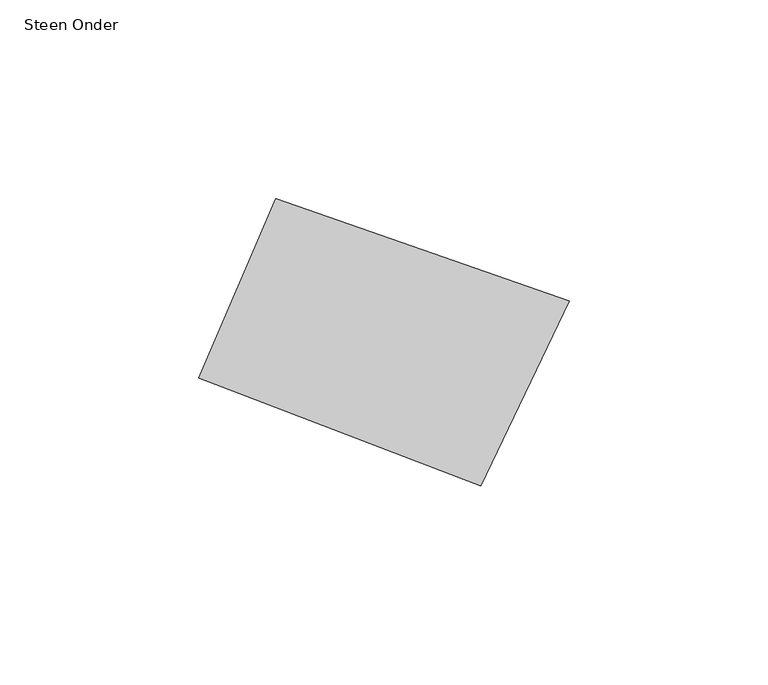
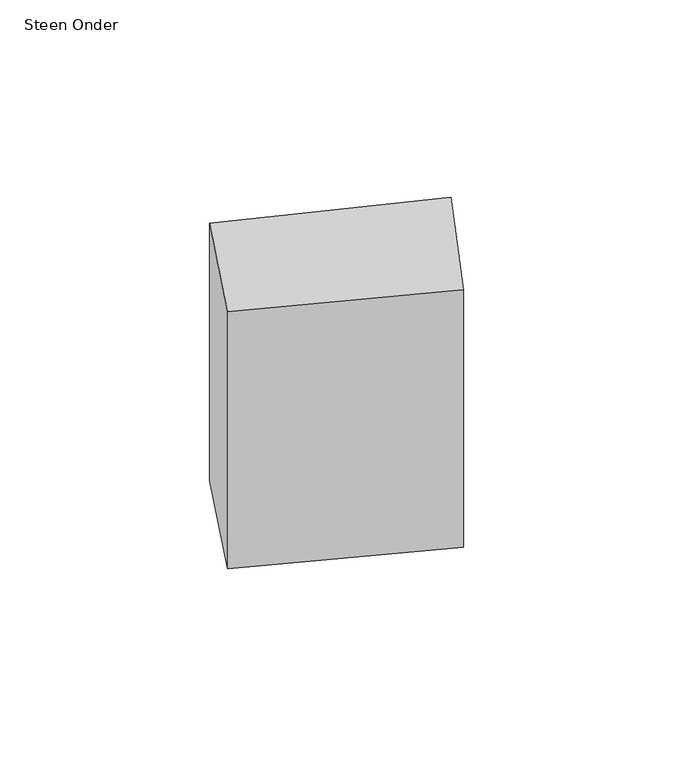
"""IFC4 building model written with IfcOpenShell, lengths in millimetres: proxy geometry, 00_GMA_steen_versie_4 : Steen Onder."""

from ifc_helpers import new_model, si_unit, frame, origin, place, context, project, spatial, polyline, outline, extrude, source, transform, mapped, element, save


def steen_onder_1c1f4d6d(model_context):
    return source(origin(), model_context, "Body", "SweptSolid", [
        extrude(outline(polyline([(138.2153403, 51.911045), (115.9401022, 5.2313815), (44.8164561, 32.4357612), (64.2804449, 77.7242813), (138.2153403, 51.911045)])), frame((0.0, 0.0, -100.0), z_axis=(0.0, 0.0, 1.0), x_axis=(1.0, 0.0, 0.0)), (0.0, 0.0, 1.0), 100.0),
    ])


if __name__ == "__main__":
    model = new_model("IFC4")
    model_context = context("Model", 3, world=origin())
    ifc_project = project(units=[si_unit("LENGTHUNIT", "METRE", prefix="MILLI")], contexts=[model_context])
    site = spatial("IfcSite", under=ifc_project)
    building = spatial("IfcBuilding", under=site)
    placement = place(None, origin())
    steen_onder_shape = steen_onder_1c1f4d6d(model_context)
    element("IfcBuildingElementProxy", 1, Name="00_GMA_steen_versie_4 : Steen Onder", ObjectType="00_GMA_steen_versie_4 : Steen Onder", at=placement, inside=building, context=model_context, shape_type="MappedRepresentation", body=[
        mapped(steen_onder_shape, transform((0.0, 0.0, 0.0), x_axis=(1.0, 0.0, 0.0), y_axis=(0.0, 1.0, 0.0), z_axis=(0.0, 0.0, 1.0))),
    ])
    save(model, "model.ifc")

# Revit data of these elements
# Type "00_GMA_steen_versie_4 : Steen Onder"
#   StootVoegHalfBoven [instance default] = 5 mm
#   StootVoegHalf [instance default] = 5 mm
#   StootVoegBreedteOnder = 10 mm
#   StootVoegBreedteBoven = 10 mm
#   Steendikte = 100 mm
#   LintVoegOnderHalf = 0 mm
#   LintVoegOnder = 0 mm
#   LintVoegBovenHalf = 5 mm
#   LintVoegBoven = 10 mm
#   materiaal = none
#   MateriaalVoeg = none
#   Default Elevation = 0
